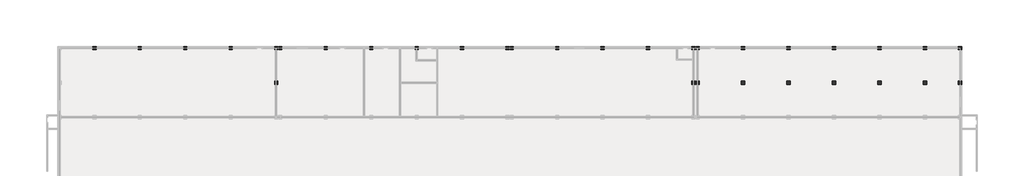
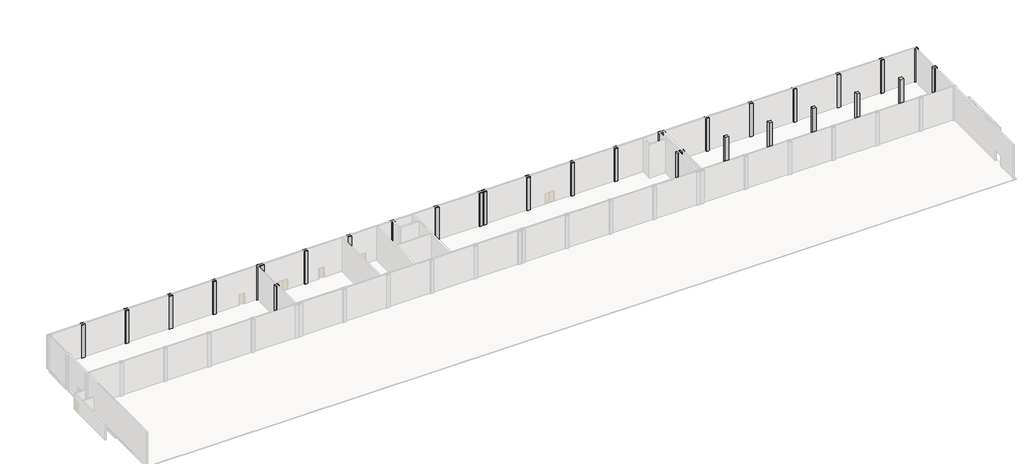
# One storey, part 4 of 4: 32 columns, 25 beams.
"""IFC4 building model written with IfcOpenShell, lengths in millimetres."""

from ifc_helpers import new_model, si_unit, frame, origin, place, context, project, spatial, polyline, outline, extrude, faceted_brep, element, save

model = new_model("IFC4")

# Units and contexts
model_context = context("Model", 3, world=origin())
ifc_project = project(units=[si_unit("LENGTHUNIT", "METRE", prefix="MILLI")], contexts=[model_context])

# Site, building, storey
site = spatial("IfcSite", under=ifc_project)
building = spatial("IfcBuilding", under=site)
storey = spatial("IfcBuildingStorey", under=building, Name="01_T.O.F", Elevation=299.9618634)

# Beams
placement = place(None, origin())
element("IfcBeam", 1, ObjectType="RC Beam_Rectangular : H_SB_AR_S16_TG_B400xH600", at=placement, inside=storey, context=model_context, shape_type="SweptSolid", body=[
    extrude(outline(polyline([(158305.0, 549.5208589), (157955.0, 549.5208589), (157955.0, 6199.5208589), (158305.0, 6199.5208589), (158305.0, 549.5208589)])), frame((0.0, 0.0, -300.0381366), z_axis=(0.0, 0.0, 1.0), x_axis=(1.0, 0.0, 0.0)), (0.0, 0.0, 1.0), 450.0),
])
element("IfcBeam", 2, ObjectType="RC Beam_Rectangular : H_SB_AR_S16_TG_B400xH600", at=placement, inside=storey, context=model_context, shape_type="SweptSolid", body=[
    extrude(outline(polyline([(157955.0, -50.4791411), (158305.0, -50.4791411), (158305.0, -5700.4791411), (157955.0, -5700.4791411), (157955.0, -50.4791411)])), frame((0.0, 0.0, -300.0381366), z_axis=(0.0, 0.0, 1.0), x_axis=(1.0, 0.0, 0.0)), (0.0, 0.0, 1.0), 450.0),
])
element("IfcBeam", 3, ObjectType="RC Beam_Rectangular : H_SB_AR_S16_TG_B400xH600", at=placement, inside=storey, context=model_context, shape_type="SweptSolid", body=[
    extrude(outline(polyline([(-4070.0, 6324.5208589), (-4070.0, 6674.5208589), (1630.0, 6674.5208589), (1630.0, 6324.5208589), (-4070.0, 6324.5208589)])), frame((0.0, 0.0, -300.0381366), z_axis=(0.0, 0.0, 1.0), x_axis=(1.0, 0.0, 0.0)), (0.0, 0.0, 1.0), 450.0),
])
element("IfcBeam", 4, ObjectType="RC Beam_Rectangular : H_SB_AR_S16_TG_B400xH600", at=placement, inside=storey, context=model_context, shape_type="SweptSolid", body=[
    extrude(outline(polyline([(2230.0, 6324.5208589), (2230.0, 6674.5208589), (9830.0, 6674.5208589), (9830.0, 6324.5208589), (2230.0, 6324.5208589)])), frame((0.0, 0.0, -300.0381366), z_axis=(0.0, 0.0, 1.0), x_axis=(1.0, 0.0, 0.0)), (0.0, 0.0, 1.0), 450.0),
])
element("IfcBeam", 5, ObjectType="RC Beam_Rectangular : H_SB_AR_S16_TG_B400xH600", at=placement, inside=storey, context=model_context, shape_type="SweptSolid", body=[
    extrude(outline(polyline([(10430.0, 6324.5208589), (10430.0, 6674.5208589), (18030.0, 6674.5208589), (18030.0, 6324.5208589), (10430.0, 6324.5208589)])), frame((0.0, 0.0, -300.0381366), z_axis=(0.0, 0.0, 1.0), x_axis=(1.0, 0.0, 0.0)), (0.0, 0.0, 1.0), 450.0),
])
element("IfcBeam", 6, ObjectType="RC Beam_Rectangular : H_SB_AR_S16_TG_B400xH600", at=placement, inside=storey, context=model_context, shape_type="SweptSolid", body=[
    extrude(outline(polyline([(18630.0, 6324.5208589), (18630.0, 6674.5208589), (26230.0, 6674.5208589), (26230.0, 6324.5208589), (18630.0, 6324.5208589)])), frame((0.0, 0.0, -300.0381366), z_axis=(0.0, 0.0, 1.0), x_axis=(1.0, 0.0, 0.0)), (0.0, 0.0, 1.0), 450.0),
])
element("IfcBeam", 7, ObjectType="RC Beam_Rectangular : H_SB_AR_S16_TG_B400xH600", at=placement, inside=storey, context=model_context, shape_type="SweptSolid", body=[
    extrude(outline(polyline([(26830.0, 6324.5208589), (26830.0, 6674.5208589), (34430.0, 6674.5208589), (34430.0, 6324.5208589), (26830.0, 6324.5208589)])), frame((0.0, 0.0, -300.0381366), z_axis=(0.0, 0.0, 1.0), x_axis=(1.0, 0.0, 0.0)), (0.0, 0.0, 1.0), 450.0),
])
element("IfcBeam", 8, ObjectType="RC Beam_Rectangular : H_SB_AR_S16_TG_B400xH600", at=placement, inside=storey, context=model_context, shape_type="SweptSolid", body=[
    extrude(outline(polyline([(35030.0, 6324.5208589), (35030.0, 6674.5208589), (35180.0, 6674.5208589), (35180.0, 6324.5208589), (35030.0, 6324.5208589)])), frame((0.0, 0.0, -300.0381366), z_axis=(0.0, 0.0, 1.0), x_axis=(1.0, 0.0, 0.0)), (0.0, 0.0, 1.0), 450.0),
])
element("IfcBeam", 9, ObjectType="RC Beam_Rectangular : H_SB_AR_S16_TG_B400xH600", at=placement, inside=storey, context=model_context, shape_type="SweptSolid", body=[
    extrude(outline(polyline([(35780.0, 6324.5208589), (35780.0, 6674.5208589), (43380.0, 6674.5208589), (43380.0, 6324.5208589), (35780.0, 6324.5208589)])), frame((0.0, 0.0, -300.0381366), z_axis=(0.0, 0.0, 1.0), x_axis=(1.0, 0.0, 0.0)), (0.0, 0.0, 1.0), 450.0),
])
element("IfcBeam", 10, ObjectType="RC Beam_Rectangular : H_SB_AR_S16_TG_B400xH600", at=placement, inside=storey, context=model_context, shape_type="SweptSolid", body=[
    extrude(outline(polyline([(43980.0, 6324.5208589), (43980.0, 6674.5208589), (51580.0, 6674.5208589), (51580.0, 6324.5208589), (43980.0, 6324.5208589)])), frame((0.0, 0.0, -300.0381366), z_axis=(0.0, 0.0, 1.0), x_axis=(1.0, 0.0, 0.0)), (0.0, 0.0, 1.0), 450.0),
])
element("IfcBeam", 11, ObjectType="RC Beam_Rectangular : H_SB_AR_S16_TG_B400xH600", at=placement, inside=storey, context=model_context, shape_type="SweptSolid", body=[
    extrude(outline(polyline([(52180.0, 6324.5208589), (52180.0, 6674.5208589), (59780.0, 6674.5208589), (59780.0, 6324.5208589), (52180.0, 6324.5208589)])), frame((0.0, 0.0, -300.0381366), z_axis=(0.0, 0.0, 1.0), x_axis=(1.0, 0.0, 0.0)), (0.0, 0.0, 1.0), 450.0),
])
element("IfcBeam", 12, ObjectType="RC Beam_Rectangular : H_SB_AR_S16_TG_B400xH600", at=placement, inside=storey, context=model_context, shape_type="SweptSolid", body=[
    extrude(outline(polyline([(60380.0, 6324.5208589), (60380.0, 6674.5208589), (67980.0, 6674.5208589), (67980.0, 6324.5208589), (60380.0, 6324.5208589)])), frame((0.0, 0.0, -300.0381366), z_axis=(0.0, 0.0, 1.0), x_axis=(1.0, 0.0, 0.0)), (0.0, 0.0, 1.0), 450.0),
])
element("IfcBeam", 13, ObjectType="RC Beam_Rectangular : H_SB_AR_S16_TG_B400xH600", at=placement, inside=storey, context=model_context, shape_type="SweptSolid", body=[
    extrude(outline(polyline([(68580.0, 6324.5208589), (68580.0, 6674.5208589), (76180.0, 6674.5208589), (76180.0, 6324.5208589), (68580.0, 6324.5208589)])), frame((0.0, 0.0, -300.0381366), z_axis=(0.0, 0.0, 1.0), x_axis=(1.0, 0.0, 0.0)), (0.0, 0.0, 1.0), 450.0),
])
element("IfcBeam", 14, ObjectType="RC Beam_Rectangular : H_SB_AR_S16_TG_B400xH600", at=placement, inside=storey, context=model_context, shape_type="SweptSolid", body=[
    extrude(outline(polyline([(76780.0, 6324.5208589), (76780.0, 6674.5208589), (76930.0, 6674.5208589), (76930.0, 6324.5208589), (76780.0, 6324.5208589)])), frame((0.0, 0.0, -300.0381366), z_axis=(0.0, 0.0, 1.0), x_axis=(1.0, 0.0, 0.0)), (0.0, 0.0, 1.0), 450.0),
])
element("IfcBeam", 15, ObjectType="RC Beam_Rectangular : H_SB_AR_S16_TG_B400xH600", at=placement, inside=storey, context=model_context, shape_type="SweptSolid", body=[
    extrude(outline(polyline([(77530.0, 6324.5208589), (77530.0, 6674.5208589), (85130.0, 6674.5208589), (85130.0, 6324.5208589), (77530.0, 6324.5208589)])), frame((0.0, 0.0, -300.0381366), z_axis=(0.0, 0.0, 1.0), x_axis=(1.0, 0.0, 0.0)), (0.0, 0.0, 1.0), 450.0),
])
element("IfcBeam", 16, ObjectType="RC Beam_Rectangular : H_SB_AR_S16_TG_B400xH600", at=placement, inside=storey, context=model_context, shape_type="SweptSolid", body=[
    extrude(outline(polyline([(85730.0, 6324.5208589), (85730.0, 6674.5208589), (93330.0, 6674.5208589), (93330.0, 6324.5208589), (85730.0, 6324.5208589)])), frame((0.0, 0.0, -300.0381366), z_axis=(0.0, 0.0, 1.0), x_axis=(1.0, 0.0, 0.0)), (0.0, 0.0, 1.0), 450.0),
])
element("IfcBeam", 17, ObjectType="RC Beam_Rectangular : H_SB_AR_S16_TG_B400xH600", at=placement, inside=storey, context=model_context, shape_type="SweptSolid", body=[
    extrude(outline(polyline([(93930.0, 6324.5208589), (93930.0, 6674.5208589), (101530.0, 6674.5208589), (101530.0, 6324.5208589), (93930.0, 6324.5208589)])), frame((0.0, 0.0, -300.0381366), z_axis=(0.0, 0.0, 1.0), x_axis=(1.0, 0.0, 0.0)), (0.0, 0.0, 1.0), 450.0),
])
element("IfcBeam", 18, ObjectType="RC Beam_Rectangular : H_SB_AR_S16_TG_B400xH600", at=placement, inside=storey, context=model_context, shape_type="SweptSolid", body=[
    extrude(outline(polyline([(102130.0, 6324.5208589), (102130.0, 6674.5208589), (109730.0, 6674.5208589), (109730.0, 6324.5208589), (102130.0, 6324.5208589)])), frame((0.0, 0.0, -300.0381366), z_axis=(0.0, 0.0, 1.0), x_axis=(1.0, 0.0, 0.0)), (0.0, 0.0, 1.0), 450.0),
])
element("IfcBeam", 19, ObjectType="RC Beam_Rectangular : H_SB_AR_S16_TG_B400xH600", at=placement, inside=storey, context=model_context, shape_type="SweptSolid", body=[
    extrude(outline(polyline([(110330.0, 6324.5208589), (110330.0, 6674.5208589), (110480.0, 6674.5208589), (110480.0, 6324.5208589), (110330.0, 6324.5208589)])), frame((0.0, 0.0, -300.0381366), z_axis=(0.0, 0.0, 1.0), x_axis=(1.0, 0.0, 0.0)), (0.0, 0.0, 1.0), 450.0),
])
element("IfcBeam", 20, ObjectType="RC Beam_Rectangular : H_SB_AR_S16_TG_B400xH600", at=placement, inside=storey, context=model_context, shape_type="SweptSolid", body=[
    extrude(outline(polyline([(111080.0, 6324.5208589), (111080.0, 6674.5208589), (118680.0, 6674.5208589), (118680.0, 6324.5208589), (111080.0, 6324.5208589)])), frame((0.0, 0.0, -300.0381366), z_axis=(0.0, 0.0, 1.0), x_axis=(1.0, 0.0, 0.0)), (0.0, 0.0, 1.0), 450.0),
])
element("IfcBeam", 21, ObjectType="RC Beam_Rectangular : H_SB_AR_S16_TG_B400xH600", at=placement, inside=storey, context=model_context, shape_type="SweptSolid", body=[
    extrude(outline(polyline([(119280.0, 6324.5208589), (119280.0, 6674.5208589), (126880.0, 6674.5208589), (126880.0, 6324.5208589), (119280.0, 6324.5208589)])), frame((0.0, 0.0, -300.0381366), z_axis=(0.0, 0.0, 1.0), x_axis=(1.0, 0.0, 0.0)), (0.0, 0.0, 1.0), 450.0),
])
element("IfcBeam", 22, ObjectType="RC Beam_Rectangular : H_SB_AR_S16_TG_B400xH600", at=placement, inside=storey, context=model_context, shape_type="SweptSolid", body=[
    extrude(outline(polyline([(127480.0, 6324.5208589), (127480.0, 6674.5208589), (135080.0, 6674.5208589), (135080.0, 6324.5208589), (127480.0, 6324.5208589)])), frame((0.0, 0.0, -300.0381366), z_axis=(0.0, 0.0, 1.0), x_axis=(1.0, 0.0, 0.0)), (0.0, 0.0, 1.0), 450.0),
])
element("IfcBeam", 23, ObjectType="RC Beam_Rectangular : H_SB_AR_S16_TG_B400xH600", at=placement, inside=storey, context=model_context, shape_type="SweptSolid", body=[
    extrude(outline(polyline([(135680.0, 6324.5208589), (135680.0, 6674.5208589), (143280.0, 6674.5208589), (143280.0, 6324.5208589), (135680.0, 6324.5208589)])), frame((0.0, 0.0, -300.0381366), z_axis=(0.0, 0.0, 1.0), x_axis=(1.0, 0.0, 0.0)), (0.0, 0.0, 1.0), 450.0),
])
element("IfcBeam", 24, ObjectType="RC Beam_Rectangular : H_SB_AR_S16_TG_B400xH600", at=placement, inside=storey, context=model_context, shape_type="SweptSolid", body=[
    extrude(outline(polyline([(143880.0, 6324.5208589), (143880.0, 6674.5208589), (151480.0, 6674.5208589), (151480.0, 6324.5208589), (143880.0, 6324.5208589)])), frame((0.0, 0.0, -300.0381366), z_axis=(0.0, 0.0, 1.0), x_axis=(1.0, 0.0, 0.0)), (0.0, 0.0, 1.0), 450.0),
])
element("IfcBeam", 25, ObjectType="RC Beam_Rectangular : H_SB_AR_S16_TG_B400xH600", at=placement, inside=storey, context=model_context, shape_type="SweptSolid", body=[
    extrude(outline(polyline([(152080.0, 6324.5208589), (152080.0, 6674.5208589), (157830.0, 6674.5208589), (157830.0, 6324.5208589), (152080.0, 6324.5208589)])), frame((0.0, 0.0, -300.0381366), z_axis=(0.0, 0.0, 1.0), x_axis=(1.0, 0.0, 0.0)), (0.0, 0.0, 1.0), 450.0),
])

# Columns
element("IfcColumn", 26, ObjectType="RC_Column_Rectangular : H_SC_AR_S15_W600xL600", at=placement, inside=storey, context=model_context, shape_type="Brep", body=[
    faceted_brep([(35030.0, 549.5208589, 299.9618634), (35030.0, -50.4791411, 299.9618634), (34430.0, -50.4791411, 299.9618634), (34430.0, 549.5208589, 299.9618634), (35030.0, 549.5208589, 6848.9618634), (35030.0, 399.5208589, 6848.9618634), (35030.0, 99.5208589, 6848.9618634), (35030.0, -50.4791411, 6848.9618634), (34880.0, -50.4791411, 6848.9618634), (34580.0, -50.4791411, 6848.9618634), (34430.0, -50.4791411, 6848.9618634), (34430.0, 99.5208589, 6848.9618634), (34430.0, 399.5208589, 6848.9618634), (34430.0, 549.5208589, 6848.9618634), (34580.0, 549.5208589, 6848.9618634), (34880.0, 549.5208589, 6848.9618634)], [[[0, 1, 2, 3]], [[1, 0, 4, 5, 6, 7]], [[2, 1, 7, 8, 9, 10]], [[3, 2, 10, 11, 12, 13]], [[0, 3, 13, 14, 15, 4]], [[7, 6, 5, 4, 15, 14, 13, 12, 11, 10, 9, 8]]]),
])
element("IfcColumn", 27, ObjectType="RC_Column_Rectangular : H_SC_AR_S15_W600xL600", at=placement, inside=storey, context=model_context, shape_type="Brep", body=[
    faceted_brep([(110330.0, 549.5208589, 299.9618634), (110330.0, -50.4791411, 299.9618634), (109730.0, -50.4791411, 299.9618634), (109730.0, 549.5208589, 299.9618634), (110330.0, 549.5208589, 6848.9618634), (110330.0, 399.5208589, 6848.9618634), (110330.0, 99.5208589, 6848.9618634), (110330.0, -50.4791411, 6848.9618634), (110180.0, -50.4791411, 6848.9618634), (109880.0, -50.4791411, 6848.9618634), (109730.0, -50.4791411, 6848.9618634), (109730.0, 99.5208589, 6848.9618634), (109730.0, 399.5208589, 6848.9618634), (109730.0, 549.5208589, 6848.9618634), (109880.0, 549.5208589, 6848.9618634), (110180.0, 549.5208589, 6848.9618634)], [[[0, 1, 2, 3]], [[1, 0, 4, 5, 6, 7]], [[2, 1, 7, 8, 9, 10]], [[3, 2, 10, 11, 12, 13]], [[0, 3, 13, 14, 15, 4]], [[7, 6, 5, 4, 15, 14, 13, 12, 11, 10, 9, 8]]]),
])
element("IfcColumn", 28, ObjectType="RC_Column_Rectangular : H_SC_AR_S15_W600xL600", at=placement, inside=storey, context=model_context, shape_type="Brep", body=[
    faceted_brep([(111080.0, 549.5208589, 299.9618634), (111080.0, -50.4791411, 299.9618634), (110480.0, -50.4791411, 299.9618634), (110480.0, 549.5208589, 299.9618634), (111080.0, 549.5208589, 6848.9618634), (111080.0, 399.5208589, 6848.9618634), (111080.0, 99.5208589, 6848.9618634), (111080.0, -50.4791411, 6848.9618634), (110930.0, -50.4791411, 6848.9618634), (110630.0, -50.4791411, 6848.9618634), (110480.0, -50.4791411, 6848.9618634), (110480.0, 99.5208589, 6848.9618634), (110480.0, 399.5208589, 6848.9618634), (110480.0, 549.5208589, 6848.9618634), (110630.0, 549.5208589, 6848.9618634), (110930.0, 549.5208589, 6848.9618634)], [[[0, 1, 2, 3]], [[1, 0, 4, 5, 6, 7]], [[2, 1, 7, 8, 9, 10]], [[3, 2, 10, 11, 12, 13]], [[0, 3, 13, 14, 15, 4]], [[7, 6, 5, 4, 15, 14, 13, 12, 11, 10, 9, 8]]]),
])
element("IfcColumn", 29, ObjectType="RC_Column_Rectangular : H_SC_AR_S15_W600xL600", at=placement, inside=storey, context=model_context, shape_type="Brep", body=[
    faceted_brep([(119280.0, 549.5208589, 299.9618634), (119280.0, -50.4791411, 299.9618634), (118680.0, -50.4791411, 299.9618634), (118680.0, 549.5208589, 299.9618634), (119280.0, 549.5208589, 6848.9618634), (119280.0, 399.5208589, 6848.9618634), (119280.0, 99.5208589, 6848.9618634), (119280.0, -50.4791411, 6848.9618634), (119130.0, -50.4791411, 6848.9618634), (118830.0, -50.4791411, 6848.9618634), (118680.0, -50.4791411, 6848.9618634), (118680.0, 99.5208589, 6848.9618634), (118680.0, 399.5208589, 6848.9618634), (118680.0, 549.5208589, 6848.9618634), (118830.0, 549.5208589, 6848.9618634), (119130.0, 549.5208589, 6848.9618634)], [[[0, 1, 2, 3]], [[1, 0, 4, 5, 6, 7]], [[2, 1, 7, 8, 9, 10]], [[3, 2, 10, 11, 12, 13]], [[0, 3, 13, 14, 15, 4]], [[7, 6, 5, 4, 15, 14, 13, 12, 11, 10, 9, 8]]]),
])
element("IfcColumn", 30, ObjectType="RC_Column_Rectangular : H_SC_AR_S15_W600xL600", at=placement, inside=storey, context=model_context, shape_type="Brep", body=[
    faceted_brep([(127480.0, 549.5208589, 299.9618634), (127480.0, -50.4791411, 299.9618634), (126880.0, -50.4791411, 299.9618634), (126880.0, 549.5208589, 299.9618634), (127480.0, 549.5208589, 6848.9618634), (127480.0, 399.5208589, 6848.9618634), (127480.0, 99.5208589, 6848.9618634), (127480.0, -50.4791411, 6848.9618634), (127330.0, -50.4791411, 6848.9618634), (127030.0, -50.4791411, 6848.9618634), (126880.0, -50.4791411, 6848.9618634), (126880.0, 99.5208589, 6848.9618634), (126880.0, 399.5208589, 6848.9618634), (126880.0, 549.5208589, 6848.9618634), (127030.0, 549.5208589, 6848.9618634), (127330.0, 549.5208589, 6848.9618634)], [[[0, 1, 2, 3]], [[1, 0, 4, 5, 6, 7]], [[2, 1, 7, 8, 9, 10]], [[3, 2, 10, 11, 12, 13]], [[0, 3, 13, 14, 15, 4]], [[7, 6, 5, 4, 15, 14, 13, 12, 11, 10, 9, 8]]]),
])
element("IfcColumn", 31, ObjectType="RC_Column_Rectangular : H_SC_AR_S15_W600xL600", at=placement, inside=storey, context=model_context, shape_type="Brep", body=[
    faceted_brep([(135680.0, 549.5208589, 299.9618634), (135680.0, -50.4791411, 299.9618634), (135080.0, -50.4791411, 299.9618634), (135080.0, 549.5208589, 299.9618634), (135680.0, 549.5208589, 6848.9618634), (135680.0, 399.5208589, 6848.9618634), (135680.0, 99.5208589, 6848.9618634), (135680.0, -50.4791411, 6848.9618634), (135530.0, -50.4791411, 6848.9618634), (135230.0, -50.4791411, 6848.9618634), (135080.0, -50.4791411, 6848.9618634), (135080.0, 99.5208589, 6848.9618634), (135080.0, 399.5208589, 6848.9618634), (135080.0, 549.5208589, 6848.9618634), (135230.0, 549.5208589, 6848.9618634), (135530.0, 549.5208589, 6848.9618634)], [[[0, 1, 2, 3]], [[1, 0, 4, 5, 6, 7]], [[2, 1, 7, 8, 9, 10]], [[3, 2, 10, 11, 12, 13]], [[0, 3, 13, 14, 15, 4]], [[7, 6, 5, 4, 15, 14, 13, 12, 11, 10, 9, 8]]]),
])
element("IfcColumn", 32, ObjectType="RC_Column_Rectangular : H_SC_AR_S15_W600xL600", at=placement, inside=storey, context=model_context, shape_type="Brep", body=[
    faceted_brep([(143880.0, 549.5208589, 299.9618634), (143880.0, -50.4791411, 299.9618634), (143280.0, -50.4791411, 299.9618634), (143280.0, 549.5208589, 299.9618634), (143880.0, 549.5208589, 6848.9618634), (143880.0, 399.5208589, 6848.9618634), (143880.0, 99.5208589, 6848.9618634), (143880.0, -50.4791411, 6848.9618634), (143730.0, -50.4791411, 6848.9618634), (143430.0, -50.4791411, 6848.9618634), (143280.0, -50.4791411, 6848.9618634), (143280.0, 99.5208589, 6848.9618634), (143280.0, 399.5208589, 6848.9618634), (143280.0, 549.5208589, 6848.9618634), (143430.0, 549.5208589, 6848.9618634), (143730.0, 549.5208589, 6848.9618634)], [[[0, 1, 2, 3]], [[1, 0, 4, 5, 6, 7]], [[2, 1, 7, 8, 9, 10]], [[3, 2, 10, 11, 12, 13]], [[0, 3, 13, 14, 15, 4]], [[7, 6, 5, 4, 15, 14, 13, 12, 11, 10, 9, 8]]]),
])
element("IfcColumn", 33, ObjectType="RC_Column_Rectangular : H_SC_AR_S15_W600xL600", at=placement, inside=storey, context=model_context, shape_type="Brep", body=[
    faceted_brep([(152080.0, 549.5208589, 299.9618634), (152080.0, -50.4791411, 299.9618634), (151480.0, -50.4791411, 299.9618634), (151480.0, 549.5208589, 299.9618634), (152080.0, 549.5208589, 6848.9618634), (152080.0, 399.5208589, 6848.9618634), (152080.0, 99.5208589, 6848.9618634), (152080.0, -50.4791411, 6848.9618634), (151930.0, -50.4791411, 6848.9618634), (151630.0, -50.4791411, 6848.9618634), (151480.0, -50.4791411, 6848.9618634), (151480.0, 99.5208589, 6848.9618634), (151480.0, 399.5208589, 6848.9618634), (151480.0, 549.5208589, 6848.9618634), (151630.0, 549.5208589, 6848.9618634), (151930.0, 549.5208589, 6848.9618634)], [[[0, 1, 2, 3]], [[1, 0, 4, 5, 6, 7]], [[2, 1, 7, 8, 9, 10]], [[3, 2, 10, 11, 12, 13]], [[0, 3, 13, 14, 15, 4]], [[7, 6, 5, 4, 15, 14, 13, 12, 11, 10, 9, 8]]]),
])
element("IfcColumn", 34, ObjectType="RC_Column_Rectangular : H_SC_AR_S15_W600xL600", at=placement, inside=storey, context=model_context, shape_type="Brep", body=[
    faceted_brep([(158430.0, 549.5208589, 299.9618634), (158430.0, -50.4791411, 299.9618634), (157830.0, -50.4791411, 299.9618634), (157830.0, 549.5208589, 299.9618634), (158430.0, 549.5208589, 6848.9618634), (158430.0, -50.4791411, 6848.9618634), (158280.0, -50.4791411, 6848.9618634), (157980.0, -50.4791411, 6848.9618634), (157830.0, -50.4791411, 6848.9618634), (157830.0, 99.5208589, 6848.9618634), (157830.0, 399.5208589, 6848.9618634), (157830.0, 549.5208589, 6848.9618634), (157980.0, 549.5208589, 6848.9618634), (158280.0, 549.5208589, 6848.9618634)], [[[0, 1, 2, 3]], [[1, 0, 4, 5]], [[2, 1, 5, 6, 7, 8]], [[3, 2, 8, 9, 10, 11]], [[0, 3, 11, 12, 13, 4]], [[5, 4, 13, 12, 11, 10, 9, 8, 7, 6]]]),
])
element("IfcColumn", 35, ObjectType="RC_Column_Rectangular : H_SC_AR_S15_W600xL600", at=placement, inside=storey, context=model_context, shape_type="Brep", body=[
    faceted_brep([(2230.0, 6799.5208589, 299.9618634), (2230.0, 6199.5208589, 299.9618634), (1630.0, 6199.5208589, 299.9618634), (1630.0, 6799.5208589, 299.9618634), (2230.0, 6799.5208589, 6848.9618634), (2230.0, 6649.5208589, 6848.9618634), (2230.0, 6349.5208589, 6848.9618634), (2230.0, 6199.5208589, 6848.9618634), (2080.0, 6199.5208589, 6848.9618634), (1780.0, 6199.5208589, 6848.9618634), (1630.0, 6199.5208589, 6848.9618634), (1630.0, 6349.5208589, 6848.9618634), (1630.0, 6649.5208589, 6848.9618634), (1630.0, 6799.5208589, 6848.9618634)], [[[0, 1, 2, 3]], [[1, 0, 4, 5, 6, 7]], [[2, 1, 7, 8, 9, 10]], [[3, 2, 10, 11, 12, 13]], [[0, 3, 13, 4]], [[7, 6, 5, 4, 13, 12, 11, 10, 9, 8]]]),
])
element("IfcColumn", 36, ObjectType="RC_Column_Rectangular : H_SC_AR_S15_W600xL600", at=placement, inside=storey, context=model_context, shape_type="Brep", body=[
    faceted_brep([(10430.0, 6799.5208589, 299.9618634), (10430.0, 6199.5208589, 299.9618634), (9830.0, 6199.5208589, 299.9618634), (9830.0, 6799.5208589, 299.9618634), (10430.0, 6799.5208589, 6848.9618634), (10430.0, 6649.5208589, 6848.9618634), (10430.0, 6349.5208589, 6848.9618634), (10430.0, 6199.5208589, 6848.9618634), (10280.0, 6199.5208589, 6848.9618634), (9980.0, 6199.5208589, 6848.9618634), (9830.0, 6199.5208589, 6848.9618634), (9830.0, 6349.5208589, 6848.9618634), (9830.0, 6649.5208589, 6848.9618634), (9830.0, 6799.5208589, 6848.9618634)], [[[0, 1, 2, 3]], [[1, 0, 4, 5, 6, 7]], [[2, 1, 7, 8, 9, 10]], [[3, 2, 10, 11, 12, 13]], [[0, 3, 13, 4]], [[7, 6, 5, 4, 13, 12, 11, 10, 9, 8]]]),
])
element("IfcColumn", 37, ObjectType="RC_Column_Rectangular : H_SC_AR_S15_W600xL600", at=placement, inside=storey, context=model_context, shape_type="Brep", body=[
    faceted_brep([(18630.0, 6799.5208589, 299.9618634), (18630.0, 6199.5208589, 299.9618634), (18030.0, 6199.5208589, 299.9618634), (18030.0, 6799.5208589, 299.9618634), (18630.0, 6799.5208589, 6848.9618634), (18630.0, 6649.5208589, 6848.9618634), (18630.0, 6349.5208589, 6848.9618634), (18630.0, 6199.5208589, 6848.9618634), (18480.0, 6199.5208589, 6848.9618634), (18180.0, 6199.5208589, 6848.9618634), (18030.0, 6199.5208589, 6848.9618634), (18030.0, 6349.5208589, 6848.9618634), (18030.0, 6649.5208589, 6848.9618634), (18030.0, 6799.5208589, 6848.9618634)], [[[0, 1, 2, 3]], [[1, 0, 4, 5, 6, 7]], [[2, 1, 7, 8, 9, 10]], [[3, 2, 10, 11, 12, 13]], [[0, 3, 13, 4]], [[7, 6, 5, 4, 13, 12, 11, 10, 9, 8]]]),
])
element("IfcColumn", 38, ObjectType="RC_Column_Rectangular : H_SC_AR_S15_W600xL600", at=placement, inside=storey, context=model_context, shape_type="Brep", body=[
    faceted_brep([(26830.0, 6799.5208589, 299.9618634), (26830.0, 6199.5208589, 299.9618634), (26230.0, 6199.5208589, 299.9618634), (26230.0, 6799.5208589, 299.9618634), (26830.0, 6799.5208589, 6848.9618634), (26830.0, 6649.5208589, 6848.9618634), (26830.0, 6349.5208589, 6848.9618634), (26830.0, 6199.5208589, 6848.9618634), (26680.0, 6199.5208589, 6848.9618634), (26380.0, 6199.5208589, 6848.9618634), (26230.0, 6199.5208589, 6848.9618634), (26230.0, 6349.5208589, 6848.9618634), (26230.0, 6649.5208589, 6848.9618634), (26230.0, 6799.5208589, 6848.9618634)], [[[0, 1, 2, 3]], [[1, 0, 4, 5, 6, 7]], [[2, 1, 7, 8, 9, 10]], [[3, 2, 10, 11, 12, 13]], [[0, 3, 13, 4]], [[7, 6, 5, 4, 13, 12, 11, 10, 9, 8]]]),
])
element("IfcColumn", 39, ObjectType="RC_Column_Rectangular : H_SC_AR_S15_W600xL600", at=placement, inside=storey, context=model_context, shape_type="Brep", body=[
    faceted_brep([(35030.0, 6799.5208589, 299.9618634), (35030.0, 6199.5208589, 299.9618634), (34430.0, 6199.5208589, 299.9618634), (34430.0, 6799.5208589, 299.9618634), (35030.0, 6799.5208589, 6848.9618634), (35030.0, 6649.5208589, 6848.9618634), (35030.0, 6349.5208589, 6848.9618634), (35030.0, 6199.5208589, 6848.9618634), (34880.0, 6199.5208589, 6848.9618634), (34580.0, 6199.5208589, 6848.9618634), (34430.0, 6199.5208589, 6848.9618634), (34430.0, 6349.5208589, 6848.9618634), (34430.0, 6649.5208589, 6848.9618634), (34430.0, 6799.5208589, 6848.9618634)], [[[0, 1, 2, 3]], [[1, 0, 4, 5, 6, 7]], [[2, 1, 7, 8, 9, 10]], [[3, 2, 10, 11, 12, 13]], [[0, 3, 13, 4]], [[7, 6, 5, 4, 13, 12, 11, 10, 9, 8]]]),
])
element("IfcColumn", 40, ObjectType="RC_Column_Rectangular : H_SC_AR_S15_W600xL600", at=placement, inside=storey, context=model_context, shape_type="Brep", body=[
    faceted_brep([(35780.0, 6799.5208589, 299.9618634), (35780.0, 6199.5208589, 299.9618634), (35180.0, 6199.5208589, 299.9618634), (35180.0, 6799.5208589, 299.9618634), (35780.0, 6799.5208589, 6848.9618634), (35780.0, 6649.5208589, 6848.9618634), (35780.0, 6349.5208589, 6848.9618634), (35780.0, 6199.5208589, 6848.9618634), (35630.0, 6199.5208589, 6848.9618634), (35330.0, 6199.5208589, 6848.9618634), (35180.0, 6199.5208589, 6848.9618634), (35180.0, 6349.5208589, 6848.9618634), (35180.0, 6649.5208589, 6848.9618634), (35180.0, 6799.5208589, 6848.9618634)], [[[0, 1, 2, 3]], [[1, 0, 4, 5, 6, 7]], [[2, 1, 7, 8, 9, 10]], [[3, 2, 10, 11, 12, 13]], [[0, 3, 13, 4]], [[7, 6, 5, 4, 13, 12, 11, 10, 9, 8]]]),
])
element("IfcColumn", 41, ObjectType="RC_Column_Rectangular : H_SC_AR_S15_W600xL600", at=placement, inside=storey, context=model_context, shape_type="Brep", body=[
    faceted_brep([(43980.0, 6799.5208589, 299.9618634), (43980.0, 6199.5208589, 299.9618634), (43380.0, 6199.5208589, 299.9618634), (43380.0, 6799.5208589, 299.9618634), (43980.0, 6799.5208589, 6848.9618634), (43980.0, 6649.5208589, 6848.9618634), (43980.0, 6349.5208589, 6848.9618634), (43980.0, 6199.5208589, 6848.9618634), (43830.0, 6199.5208589, 6848.9618634), (43530.0, 6199.5208589, 6848.9618634), (43380.0, 6199.5208589, 6848.9618634), (43380.0, 6349.5208589, 6848.9618634), (43380.0, 6649.5208589, 6848.9618634), (43380.0, 6799.5208589, 6848.9618634)], [[[0, 1, 2, 3]], [[1, 0, 4, 5, 6, 7]], [[2, 1, 7, 8, 9, 10]], [[3, 2, 10, 11, 12, 13]], [[0, 3, 13, 4]], [[7, 6, 5, 4, 13, 12, 11, 10, 9, 8]]]),
])
element("IfcColumn", 42, ObjectType="RC_Column_Rectangular : H_SC_AR_S15_W600xL600", at=placement, inside=storey, context=model_context, shape_type="Brep", body=[
    faceted_brep([(52180.0, 6799.5208589, 299.9618634), (52180.0, 6199.5208589, 299.9618634), (51580.0, 6199.5208589, 299.9618634), (51580.0, 6799.5208589, 299.9618634), (52180.0, 6799.5208589, 6848.9618634), (52180.0, 6649.5208589, 6848.9618634), (52180.0, 6349.5208589, 6848.9618634), (52180.0, 6199.5208589, 6848.9618634), (52030.0, 6199.5208589, 6848.9618634), (51730.0, 6199.5208589, 6848.9618634), (51580.0, 6199.5208589, 6848.9618634), (51580.0, 6349.5208589, 6848.9618634), (51580.0, 6649.5208589, 6848.9618634), (51580.0, 6799.5208589, 6848.9618634)], [[[0, 1, 2, 3]], [[1, 0, 4, 5, 6, 7]], [[2, 1, 7, 8, 9, 10]], [[3, 2, 10, 11, 12, 13]], [[0, 3, 13, 4]], [[7, 6, 5, 4, 13, 12, 11, 10, 9, 8]]]),
])
element("IfcColumn", 43, ObjectType="RC_Column_Rectangular : H_SC_AR_S15_W600xL600", at=placement, inside=storey, context=model_context, shape_type="Brep", body=[
    faceted_brep([(60380.0, 6799.5208589, 299.9618634), (60380.0, 6199.5208589, 299.9618634), (59780.0, 6199.5208589, 299.9618634), (59780.0, 6799.5208589, 299.9618634), (60380.0, 6799.5208589, 6848.9618634), (60380.0, 6649.5208589, 6848.9618634), (60380.0, 6349.5208589, 6848.9618634), (60380.0, 6199.5208589, 6848.9618634), (60230.0, 6199.5208589, 6848.9618634), (59930.0, 6199.5208589, 6848.9618634), (59780.0, 6199.5208589, 6848.9618634), (59780.0, 6349.5208589, 6848.9618634), (59780.0, 6649.5208589, 6848.9618634), (59780.0, 6799.5208589, 6848.9618634)], [[[0, 1, 2, 3]], [[1, 0, 4, 5, 6, 7]], [[2, 1, 7, 8, 9, 10]], [[3, 2, 10, 11, 12, 13]], [[0, 3, 13, 4]], [[7, 6, 5, 4, 13, 12, 11, 10, 9, 8]]]),
])
element("IfcColumn", 44, ObjectType="RC_Column_Rectangular : H_SC_AR_S15_W600xL600", at=placement, inside=storey, context=model_context, shape_type="Brep", body=[
    faceted_brep([(68580.0, 6799.5208589, 299.9618634), (68580.0, 6199.5208589, 299.9618634), (67980.0, 6199.5208589, 299.9618634), (67980.0, 6799.5208589, 299.9618634), (68580.0, 6799.5208589, 6848.9618634), (68580.0, 6649.5208589, 6848.9618634), (68580.0, 6349.5208589, 6848.9618634), (68580.0, 6199.5208589, 6848.9618634), (68430.0, 6199.5208589, 6848.9618634), (68130.0, 6199.5208589, 6848.9618634), (67980.0, 6199.5208589, 6848.9618634), (67980.0, 6349.5208589, 6848.9618634), (67980.0, 6649.5208589, 6848.9618634), (67980.0, 6799.5208589, 6848.9618634)], [[[0, 1, 2, 3]], [[1, 0, 4, 5, 6, 7]], [[2, 1, 7, 8, 9, 10]], [[3, 2, 10, 11, 12, 13]], [[0, 3, 13, 4]], [[7, 6, 5, 4, 13, 12, 11, 10, 9, 8]]]),
])
element("IfcColumn", 45, ObjectType="RC_Column_Rectangular : H_SC_AR_S15_W600xL600", at=placement, inside=storey, context=model_context, shape_type="Brep", body=[
    faceted_brep([(76780.0, 6799.5208589, 299.9618634), (76780.0, 6199.5208589, 299.9618634), (76180.0, 6199.5208589, 299.9618634), (76180.0, 6799.5208589, 299.9618634), (76780.0, 6799.5208589, 6848.9618634), (76780.0, 6649.5208589, 6848.9618634), (76780.0, 6349.5208589, 6848.9618634), (76780.0, 6199.5208589, 6848.9618634), (76630.0, 6199.5208589, 6848.9618634), (76330.0, 6199.5208589, 6848.9618634), (76180.0, 6199.5208589, 6848.9618634), (76180.0, 6349.5208589, 6848.9618634), (76180.0, 6649.5208589, 6848.9618634), (76180.0, 6799.5208589, 6848.9618634)], [[[0, 1, 2, 3]], [[1, 0, 4, 5, 6, 7]], [[2, 1, 7, 8, 9, 10]], [[3, 2, 10, 11, 12, 13]], [[0, 3, 13, 4]], [[7, 6, 5, 4, 13, 12, 11, 10, 9, 8]]]),
])
element("IfcColumn", 46, ObjectType="RC_Column_Rectangular : H_SC_AR_S15_W600xL600", at=placement, inside=storey, context=model_context, shape_type="Brep", body=[
    faceted_brep([(77530.0, 6799.5208589, 299.9618634), (77530.0, 6199.5208589, 299.9618634), (76930.0, 6199.5208589, 299.9618634), (76930.0, 6799.5208589, 299.9618634), (77530.0, 6799.5208589, 6848.9618634), (77530.0, 6649.5208589, 6848.9618634), (77530.0, 6349.5208589, 6848.9618634), (77530.0, 6199.5208589, 6848.9618634), (77380.0, 6199.5208589, 6848.9618634), (77080.0, 6199.5208589, 6848.9618634), (76930.0, 6199.5208589, 6848.9618634), (76930.0, 6349.5208589, 6848.9618634), (76930.0, 6649.5208589, 6848.9618634), (76930.0, 6799.5208589, 6848.9618634)], [[[0, 1, 2, 3]], [[1, 0, 4, 5, 6, 7]], [[2, 1, 7, 8, 9, 10]], [[3, 2, 10, 11, 12, 13]], [[0, 3, 13, 4]], [[7, 6, 5, 4, 13, 12, 11, 10, 9, 8]]]),
])
element("IfcColumn", 47, ObjectType="RC_Column_Rectangular : H_SC_AR_S15_W600xL600", at=placement, inside=storey, context=model_context, shape_type="Brep", body=[
    faceted_brep([(85730.0, 6799.5208589, 299.9618634), (85730.0, 6199.5208589, 299.9618634), (85130.0, 6199.5208589, 299.9618634), (85130.0, 6799.5208589, 299.9618634), (85730.0, 6799.5208589, 6848.9618634), (85730.0, 6649.5208589, 6848.9618634), (85730.0, 6349.5208589, 6848.9618634), (85730.0, 6199.5208589, 6848.9618634), (85580.0, 6199.5208589, 6848.9618634), (85280.0, 6199.5208589, 6848.9618634), (85130.0, 6199.5208589, 6848.9618634), (85130.0, 6349.5208589, 6848.9618634), (85130.0, 6649.5208589, 6848.9618634), (85130.0, 6799.5208589, 6848.9618634)], [[[0, 1, 2, 3]], [[1, 0, 4, 5, 6, 7]], [[2, 1, 7, 8, 9, 10]], [[3, 2, 10, 11, 12, 13]], [[0, 3, 13, 4]], [[7, 6, 5, 4, 13, 12, 11, 10, 9, 8]]]),
])
element("IfcColumn", 48, ObjectType="RC_Column_Rectangular : H_SC_AR_S15_W600xL600", at=placement, inside=storey, context=model_context, shape_type="Brep", body=[
    faceted_brep([(93930.0, 6799.5208589, 299.9618634), (93930.0, 6199.5208589, 299.9618634), (93330.0, 6199.5208589, 299.9618634), (93330.0, 6799.5208589, 299.9618634), (93930.0, 6799.5208589, 6848.9618634), (93930.0, 6649.5208589, 6848.9618634), (93930.0, 6349.5208589, 6848.9618634), (93930.0, 6199.5208589, 6848.9618634), (93780.0, 6199.5208589, 6848.9618634), (93480.0, 6199.5208589, 6848.9618634), (93330.0, 6199.5208589, 6848.9618634), (93330.0, 6349.5208589, 6848.9618634), (93330.0, 6649.5208589, 6848.9618634), (93330.0, 6799.5208589, 6848.9618634)], [[[0, 1, 2, 3]], [[1, 0, 4, 5, 6, 7]], [[2, 1, 7, 8, 9, 10]], [[3, 2, 10, 11, 12, 13]], [[0, 3, 13, 4]], [[7, 6, 5, 4, 13, 12, 11, 10, 9, 8]]]),
])
element("IfcColumn", 49, ObjectType="RC_Column_Rectangular : H_SC_AR_S15_W600xL600", at=placement, inside=storey, context=model_context, shape_type="Brep", body=[
    faceted_brep([(102130.0, 6799.5208589, 299.9618634), (102130.0, 6199.5208589, 299.9618634), (101530.0, 6199.5208589, 299.9618634), (101530.0, 6799.5208589, 299.9618634), (102130.0, 6799.5208589, 6848.9618634), (102130.0, 6649.5208589, 6848.9618634), (102130.0, 6349.5208589, 6848.9618634), (102130.0, 6199.5208589, 6848.9618634), (101980.0, 6199.5208589, 6848.9618634), (101680.0, 6199.5208589, 6848.9618634), (101530.0, 6199.5208589, 6848.9618634), (101530.0, 6349.5208589, 6848.9618634), (101530.0, 6649.5208589, 6848.9618634), (101530.0, 6799.5208589, 6848.9618634)], [[[0, 1, 2, 3]], [[1, 0, 4, 5, 6, 7]], [[2, 1, 7, 8, 9, 10]], [[3, 2, 10, 11, 12, 13]], [[0, 3, 13, 4]], [[7, 6, 5, 4, 13, 12, 11, 10, 9, 8]]]),
])
element("IfcColumn", 50, ObjectType="RC_Column_Rectangular : H_SC_AR_S15_W600xL600", at=placement, inside=storey, context=model_context, shape_type="Brep", body=[
    faceted_brep([(110330.0, 6799.5208589, 299.9618634), (110330.0, 6199.5208589, 299.9618634), (109730.0, 6199.5208589, 299.9618634), (109730.0, 6799.5208589, 299.9618634), (110330.0, 6799.5208589, 6848.9618634), (110330.0, 6649.5208589, 6848.9618634), (110330.0, 6349.5208589, 6848.9618634), (110330.0, 6199.5208589, 6848.9618634), (110180.0, 6199.5208589, 6848.9618634), (109880.0, 6199.5208589, 6848.9618634), (109730.0, 6199.5208589, 6848.9618634), (109730.0, 6349.5208589, 6848.9618634), (109730.0, 6649.5208589, 6848.9618634), (109730.0, 6799.5208589, 6848.9618634)], [[[0, 1, 2, 3]], [[1, 0, 4, 5, 6, 7]], [[2, 1, 7, 8, 9, 10]], [[3, 2, 10, 11, 12, 13]], [[0, 3, 13, 4]], [[7, 6, 5, 4, 13, 12, 11, 10, 9, 8]]]),
])
element("IfcColumn", 51, ObjectType="RC_Column_Rectangular : H_SC_AR_S15_W600xL600", at=placement, inside=storey, context=model_context, shape_type="Brep", body=[
    faceted_brep([(111080.0, 6799.5208589, 299.9618634), (111080.0, 6199.5208589, 299.9618634), (110480.0, 6199.5208589, 299.9618634), (110480.0, 6799.5208589, 299.9618634), (111080.0, 6799.5208589, 6848.9618634), (111080.0, 6649.5208589, 6848.9618634), (111080.0, 6349.5208589, 6848.9618634), (111080.0, 6199.5208589, 6848.9618634), (110930.0, 6199.5208589, 6848.9618634), (110630.0, 6199.5208589, 6848.9618634), (110480.0, 6199.5208589, 6848.9618634), (110480.0, 6349.5208589, 6848.9618634), (110480.0, 6649.5208589, 6848.9618634), (110480.0, 6799.5208589, 6848.9618634)], [[[0, 1, 2, 3]], [[1, 0, 4, 5, 6, 7]], [[2, 1, 7, 8, 9, 10]], [[3, 2, 10, 11, 12, 13]], [[0, 3, 13, 4]], [[7, 6, 5, 4, 13, 12, 11, 10, 9, 8]]]),
])
element("IfcColumn", 52, ObjectType="RC_Column_Rectangular : H_SC_AR_S15_W600xL600", at=placement, inside=storey, context=model_context, shape_type="Brep", body=[
    faceted_brep([(119280.0, 6799.5208589, 299.9618634), (119280.0, 6199.5208589, 299.9618634), (118680.0, 6199.5208589, 299.9618634), (118680.0, 6799.5208589, 299.9618634), (119280.0, 6799.5208589, 6848.9618634), (119280.0, 6649.5208589, 6848.9618634), (119280.0, 6349.5208589, 6848.9618634), (119280.0, 6199.5208589, 6848.9618634), (119130.0, 6199.5208589, 6848.9618634), (118830.0, 6199.5208589, 6848.9618634), (118680.0, 6199.5208589, 6848.9618634), (118680.0, 6349.5208589, 6848.9618634), (118680.0, 6649.5208589, 6848.9618634), (118680.0, 6799.5208589, 6848.9618634)], [[[0, 1, 2, 3]], [[1, 0, 4, 5, 6, 7]], [[2, 1, 7, 8, 9, 10]], [[3, 2, 10, 11, 12, 13]], [[0, 3, 13, 4]], [[7, 6, 5, 4, 13, 12, 11, 10, 9, 8]]]),
])
element("IfcColumn", 53, ObjectType="RC_Column_Rectangular : H_SC_AR_S15_W600xL600", at=placement, inside=storey, context=model_context, shape_type="Brep", body=[
    faceted_brep([(127480.0, 6799.5208589, 299.9618634), (127480.0, 6199.5208589, 299.9618634), (126880.0, 6199.5208589, 299.9618634), (126880.0, 6799.5208589, 299.9618634), (127480.0, 6799.5208589, 6848.9618634), (127480.0, 6649.5208589, 6848.9618634), (127480.0, 6349.5208589, 6848.9618634), (127480.0, 6199.5208589, 6848.9618634), (127330.0, 6199.5208589, 6848.9618634), (127030.0, 6199.5208589, 6848.9618634), (126880.0, 6199.5208589, 6848.9618634), (126880.0, 6349.5208589, 6848.9618634), (126880.0, 6649.5208589, 6848.9618634), (126880.0, 6799.5208589, 6848.9618634)], [[[0, 1, 2, 3]], [[1, 0, 4, 5, 6, 7]], [[2, 1, 7, 8, 9, 10]], [[3, 2, 10, 11, 12, 13]], [[0, 3, 13, 4]], [[7, 6, 5, 4, 13, 12, 11, 10, 9, 8]]]),
])
element("IfcColumn", 54, ObjectType="RC_Column_Rectangular : H_SC_AR_S15_W600xL600", at=placement, inside=storey, context=model_context, shape_type="Brep", body=[
    faceted_brep([(135680.0, 6799.5208589, 299.9618634), (135680.0, 6199.5208589, 299.9618634), (135080.0, 6199.5208589, 299.9618634), (135080.0, 6799.5208589, 299.9618634), (135680.0, 6799.5208589, 6848.9618634), (135680.0, 6649.5208589, 6848.9618634), (135680.0, 6349.5208589, 6848.9618634), (135680.0, 6199.5208589, 6848.9618634), (135530.0, 6199.5208589, 6848.9618634), (135230.0, 6199.5208589, 6848.9618634), (135080.0, 6199.5208589, 6848.9618634), (135080.0, 6349.5208589, 6848.9618634), (135080.0, 6649.5208589, 6848.9618634), (135080.0, 6799.5208589, 6848.9618634)], [[[0, 1, 2, 3]], [[1, 0, 4, 5, 6, 7]], [[2, 1, 7, 8, 9, 10]], [[3, 2, 10, 11, 12, 13]], [[0, 3, 13, 4]], [[7, 6, 5, 4, 13, 12, 11, 10, 9, 8]]]),
])
element("IfcColumn", 55, ObjectType="RC_Column_Rectangular : H_SC_AR_S15_W600xL600", at=placement, inside=storey, context=model_context, shape_type="Brep", body=[
    faceted_brep([(143880.0, 6799.5208589, 299.9618634), (143880.0, 6199.5208589, 299.9618634), (143280.0, 6199.5208589, 299.9618634), (143280.0, 6799.5208589, 299.9618634), (143880.0, 6799.5208589, 6848.9618634), (143880.0, 6649.5208589, 6848.9618634), (143880.0, 6349.5208589, 6848.9618634), (143880.0, 6199.5208589, 6848.9618634), (143730.0, 6199.5208589, 6848.9618634), (143430.0, 6199.5208589, 6848.9618634), (143280.0, 6199.5208589, 6848.9618634), (143280.0, 6349.5208589, 6848.9618634), (143280.0, 6649.5208589, 6848.9618634), (143280.0, 6799.5208589, 6848.9618634)], [[[0, 1, 2, 3]], [[1, 0, 4, 5, 6, 7]], [[2, 1, 7, 8, 9, 10]], [[3, 2, 10, 11, 12, 13]], [[0, 3, 13, 4]], [[7, 6, 5, 4, 13, 12, 11, 10, 9, 8]]]),
])
element("IfcColumn", 56, ObjectType="RC_Column_Rectangular : H_SC_AR_S15_W600xL600", at=placement, inside=storey, context=model_context, shape_type="Brep", body=[
    faceted_brep([(152080.0, 6799.5208589, 299.9618634), (152080.0, 6199.5208589, 299.9618634), (151480.0, 6199.5208589, 299.9618634), (151480.0, 6799.5208589, 299.9618634), (152080.0, 6799.5208589, 6848.9618634), (152080.0, 6649.5208589, 6848.9618634), (152080.0, 6349.5208589, 6848.9618634), (152080.0, 6199.5208589, 6848.9618634), (151930.0, 6199.5208589, 6848.9618634), (151630.0, 6199.5208589, 6848.9618634), (151480.0, 6199.5208589, 6848.9618634), (151480.0, 6349.5208589, 6848.9618634), (151480.0, 6649.5208589, 6848.9618634), (151480.0, 6799.5208589, 6848.9618634)], [[[0, 1, 2, 3]], [[1, 0, 4, 5, 6, 7]], [[2, 1, 7, 8, 9, 10]], [[3, 2, 10, 11, 12, 13]], [[0, 3, 13, 4]], [[7, 6, 5, 4, 13, 12, 11, 10, 9, 8]]]),
])
element("IfcColumn", 57, ObjectType="RC_Column_Rectangular : H_SC_AR_S15_W600xL600", at=placement, inside=storey, context=model_context, shape_type="Brep", body=[
    faceted_brep([(158430.0, 6799.5208589, 299.9618634), (158430.0, 6199.5208589, 299.9618634), (157830.0, 6199.5208589, 299.9618634), (157830.0, 6799.5208589, 299.9618634), (158430.0, 6799.5208589, 6848.9618634), (158430.0, 6199.5208589, 6848.9618634), (158280.0, 6199.5208589, 6848.9618634), (157980.0, 6199.5208589, 6848.9618634), (157830.0, 6199.5208589, 6848.9618634), (157830.0, 6349.5208589, 6848.9618634), (157830.0, 6649.5208589, 6848.9618634), (157830.0, 6799.5208589, 6848.9618634)], [[[0, 1, 2, 3]], [[1, 0, 4, 5]], [[2, 1, 5, 6, 7, 8]], [[3, 2, 8, 9, 10, 11]], [[0, 3, 11, 4]], [[5, 4, 11, 10, 9, 8, 7, 6]]]),
])

save(model, "model.ifc")

# Revit data of these elements
# Type "RC Beam_Rectangular : H_SB_AR_S16_TG_B400xH600"
#   중앙부 하부근 = ""
#   중앙부 상부근 = ""
#   중앙부 보조근 = ""
#   중앙부 늑근 = ""
#   외단부 하부근 = ""
#   외단부 상부근 = ""
#   외단부 보조근 = ""
#   외단부 늑근 = ""
#   부호 = "TG2"
#   내단부 하부근 = ""
#   내단부 상부근 = ""
#   내단부 보조근 = ""
#   내단부 늑근 = ""
#   ALL 하부근 = "3-D20"
#   ALL 상부근 = "4-D20"
#   ALL 보조근 = ""
#   ALL 늑근 = "2-D10 @120"
#   Width = 350 mm
#   Height = 600 mm
#   Length [instance default] = 1524 mm
#   b = 350 mm
#   h = 600 mm
#   hec_material3 [instance default] = none
#   hec_material2 [instance default] = none
#   hec_material1 [instance default] = none
#   Structural Material [instance default] = none
#   Assembly Code = ""
# Type "RC_Column_Rectangular : H_SC_AR_S15_W600xL600"
#   Width = 600 mm
#   Length = 600 mm
#   hec_material3 [instance default] = none
#   hec_material2 [instance default] = none
#   hec_material1 [instance default] = none
#   Structural Material [instance default] = none
#   Description = (empty or 0)
# Elements 1, 2, 3, 4, 5, 6, 7, 8, 9, 10, 11, 12, 13, 14, 15, 16, 17, 18, 19, 20, 21, 22, 23, 24, 25 (IfcBeam, "RC Beam_Rectangular : H_SB_AR_S16_TG_B400xH600")
#   Comments = ""
#   hec_material3 = none
#   hec_material2 = none
#   hec_material1 = none
#   Structural Material = none
#   Phase Created = New Construction
# Elements 26, 27, 28, 29, 30, 31, 32, 33, 34, 35, 36, 37, 38, 39, 40, 41, 42, 43, 44, 45, 46, 47, 48, 49, 50, 51, 52, 53, 54, 55, 56, 57 (IfcColumn, "RC_Column_Rectangular : H_SC_AR_S15_W600xL600")
#   Comments = ""
#   hec_material3 = none
#   hec_material2 = none
#   hec_material1 = none
#   Structural Material = none
#   Phase Created = New Construction
